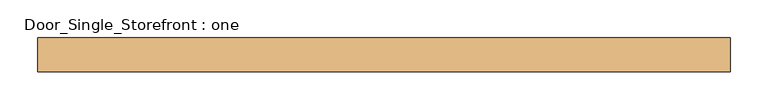
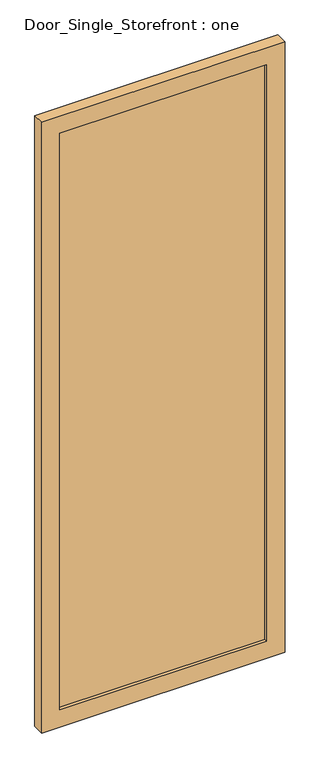
"""IFC4 building model written with IfcOpenShell, lengths in millimetres: door geometry, Door_Single_Storefront : one."""

from ifc_helpers import new_model, si_unit, frame, origin, place, context, project, spatial, polyline, outline, extrude, source, transform, mapped, element, save


def door_single_storefront_one_e0482a8f(model_context):
    return source(origin(), model_context, "Body", "SweptSolid", [
        extrude(outline(polyline([(388.9375, -6.35), (-388.9375, -6.35), (-388.9375, 12.7), (388.9375, 12.7), (388.9375, -6.35)])), frame((0.0, 0.0, 68.2625), z_axis=(0.0, 0.0, 1.0), x_axis=(1.0, 0.0, 0.0)), (0.0, 0.0, 1.0), 2289.0329118),
        extrude(outline(polyline([(2425.5579118, -457.2), (0.0, -457.2), (0.0, 457.2), (2425.5579118, 457.2), (2425.5579118, -457.2)]), holes=[polyline([(68.2625, 388.9375), (68.2625, -388.9375), (2357.2954118, -388.9375), (2357.2954118, 388.9375), (68.2625, 388.9375)])]), frame((0.0, -19.05, 0.0), z_axis=(0.0, 1.0, 0.0), x_axis=(0.0, 0.0, 1.0)), (0.0, 0.0, 1.0), 44.45),
    ])


if __name__ == "__main__":
    model = new_model("IFC4")
    model_context = context("Model", 3, world=origin())
    ifc_project = project(units=[si_unit("LENGTHUNIT", "METRE", prefix="MILLI")], contexts=[model_context])
    site = spatial("IfcSite", under=ifc_project)
    building = spatial("IfcBuilding", under=site)
    placement = place(None, origin())
    door_single_storefront_one_shape = door_single_storefront_one_e0482a8f(model_context)
    element("IfcDoor", 1, ObjectType="Door_Single_Storefront : one", at=placement, inside=building, context=model_context, shape_type="MappedRepresentation", body=[
        mapped(door_single_storefront_one_shape, transform((0.0, 0.0, 0.0), x_axis=(1.0, 0.0, 0.0), y_axis=(0.0, 1.0, 0.0), z_axis=(0.0, 0.0, 1.0))),
    ])
    save(model, "model.ifc")

# Revit data of these elements
# Type "Door_Single_Storefront : one"
#   Type Mark = "29"
#   OD_DS_Door_Material = "ALUM./GLAZING"
#   OD_DS_Door_Type = "STOREFRONT (NARROW STILE)"
#   OD_DS_Lockset = "ENTRY LOCK (INSIDE ADA LEVER ALWAYS ACTIVE)"
#   Analytic Construction = "<None>"
#   angle open [instance default] = 132.952°
#   Stile_Width = 0' - 2 11/16"
#   Door_Thickness = 0' - 1 3/4"
#   Door_Offset = 0' - 1"
#   Glass_Material = TEMPERED INSULATED GLAZING (CARDINAL GLASS LoĒ²-240\nOR EQUIVALENT)
#   Frame_Material = KAWNEER 260 INSULCLADTM THERMAL ENTRANCE - CLEAR ANODIZED ALUM.
#   Function = (empty or 0)
# Element 1 (IfcDoor, "Door_Single_Storefront : one")
#   Materials on its faces: "KAWNEER 260 INSULCLADTM THERMAL ENTRANCE - CLEAR ANODIZED ALUM.", "TEMPERED INSULATED GLAZING (CARDINAL GLASS LoĒ²-240\nOR EQUIVALENT)"
# Materials
#   "TEMPERED INSULATED GLAZING (CARDINAL GLASS LoĒ²-240\nOR EQUIVALENT)": class "Glass", colour RGB 196 205 210, transparency 0.85, Description = "Soda Lime Glass", Cost = 0
#   "KAWNEER 260 INSULCLADTM THERMAL ENTRANCE - CLEAR ANODIZED ALUM.": class "Metal", colour RGB 244 244 244, transparency 0, Description = "Aluminum 6061", Cost = 0
